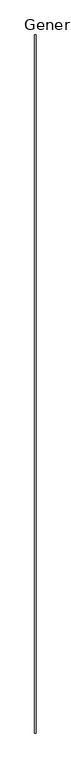
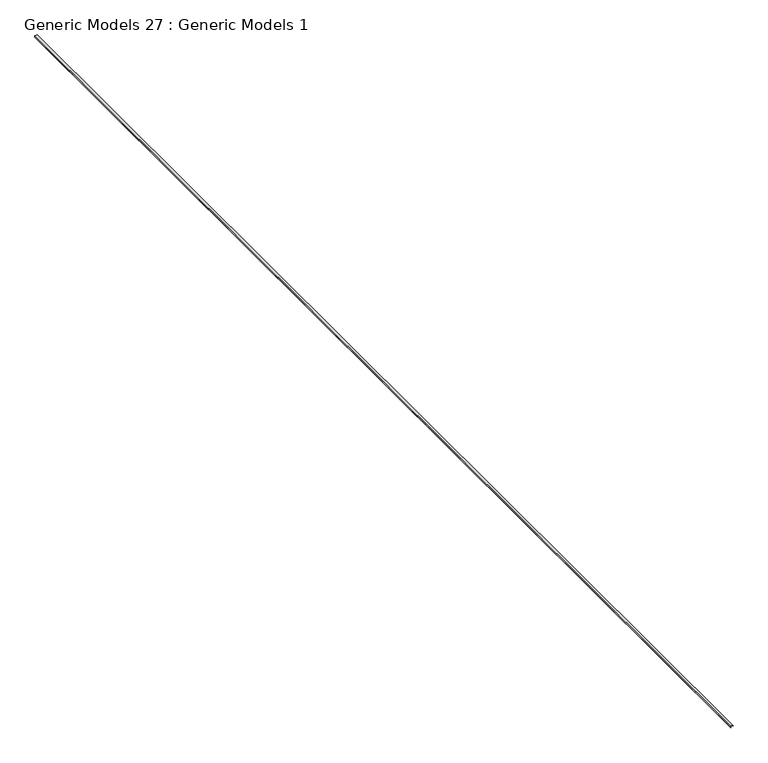
"""IFC4 building model written with IfcOpenShell, lengths in millimetres: proxy geometry, Generic Models 27 : Generic Models 1."""

from ifc_helpers import new_model, si_unit, frame, origin, place, context, project, spatial, polyline, outline, extrude, source, transform, mapped, element, save


def generic_models_27_generic_models_1_804e0e5a(model_context):
    return source(origin(), model_context, "Body", "SweptSolid", [
        extrude(outline(polyline([(126312.2670671, 8411.4566425), (126312.2670671, 8416.2064425), (126315.2695234, 8416.2064425), (126315.2695234, 8414.9364425), (126313.5370671, 8414.9364425), (126313.5370671, 8412.7266425), (126333.2220671, 8412.7266425), (126333.2220671, 8449.5566425), (126334.4920671, 8449.5566425), (126334.4920671, 8411.4566425), (126312.2670671, 8411.4566425)])), frame((0.0, -7068.1230338, 0.0), z_axis=(0.0, 1.0, 0.0), x_axis=(0.0, 0.0, 1.0)), (0.0, 0.0, 1.0), 19050.0),
    ])


if __name__ == "__main__":
    model = new_model("IFC4")
    model_context = context("Model", 3, world=origin())
    ifc_project = project(units=[si_unit("LENGTHUNIT", "METRE", prefix="MILLI")], contexts=[model_context])
    site = spatial("IfcSite", under=ifc_project)
    building = spatial("IfcBuilding", under=site)
    placement = place(None, origin())
    generic_models_27_generic_models_1_shape = generic_models_27_generic_models_1_804e0e5a(model_context)
    element("IfcBuildingElementProxy", 1, Name="Generic Models 27 : Generic Models 1", ObjectType="Generic Models 27 : Generic Models 1", at=placement, inside=building, context=model_context, shape_type="MappedRepresentation", body=[
        mapped(generic_models_27_generic_models_1_shape, transform((0.0, 0.0, 0.0), x_axis=(1.0, 0.0, 0.0), y_axis=(0.0, 1.0, 0.0), z_axis=(0.0, 0.0, 1.0))),
    ])
    save(model, "model.ifc")

# Revit data of these elements
# Element 1 (IfcBuildingElementProxy, "Generic Models 27 : Generic Models 1")
#   Materials on its faces: "_CONTINUOUS 16 GA. COPPER  J BEAD"
# Materials
#   "_CONTINUOUS 16 GA. COPPER  J BEAD": class "Generic", colour RGB 253 192 103, transparency 0, Cost = 0
